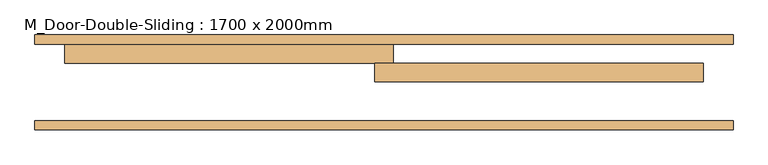
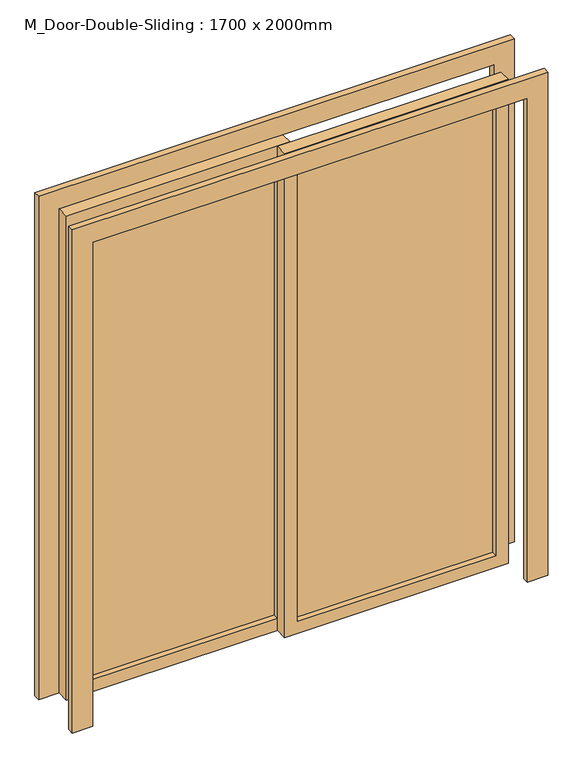
"""IFC4 building model written with IfcOpenShell, lengths in millimetres: door geometry, M_Door-Double-Sliding : 1700 x 2000mm."""

from ifc_helpers import new_model, si_unit, frame, origin, place, context, project, spatial, polyline, outline, extrude, source, transform, mapped, element, save


def m_door_double_sliding_1700_x_2000mm_96dae475(model_context):
    return source(origin(), model_context, "Body", "SweptSolid", [
        extrude(outline(polyline([(0.0, -930.0), (0.0, -850.0), (2000.0, -850.0), (2000.0, 850.0), (0.0, 850.0), (0.0, 930.0), (2080.0, 930.0), (2080.0, -930.0), (0.0, -930.0)])), frame((0.0, 0.4, 0.0), z_axis=(0.0, 1.0, 0.0), x_axis=(0.0, 0.0, 1.0)), (0.0, 0.0, 1.0), 25.0),
        extrude(outline(polyline([(0.0, 930.0), (2080.0, 930.0), (2080.0, -930.0), (0.0, -930.0), (0.0, -850.0), (2000.0, -850.0), (2000.0, 850.0), (0.0, 850.0), (0.0, 930.0)])), frame((0.0, 228.6, 0.0), z_axis=(0.0, 1.0, 0.0), x_axis=(0.0, 0.0, 1.0)), (0.0, 0.0, 1.0), 25.0),
        extrude(outline(polyline([(2000.0, -25.0), (0.0, -25.0), (0.0, 850.0), (2000.0, 850.0), (2000.0, -25.0)]), holes=[polyline([(1950.0, 25.0), (1950.0, 800.0), (50.0, 800.0), (50.0, 25.0), (1950.0, 25.0)])]), frame((0.0, 128.6, 0.0), z_axis=(0.0, 1.0, 0.0), x_axis=(0.0, 0.0, 1.0)), (0.0, 0.0, 1.0), 50.0),
        extrude(outline(polyline([(2000.0, 25.0), (2000.0, -850.0), (0.0, -850.0), (0.0, 25.0), (2000.0, 25.0)]), holes=[polyline([(1950.0, -25.0), (50.0, -25.0), (50.0, -800.0), (1950.0, -800.0), (1950.0, -25.0)])]), frame((0.0, 178.6, 0.0), z_axis=(0.0, 1.0, 0.0), x_axis=(0.0, 0.0, 1.0)), (0.0, 0.0, 1.0), 50.0),
        extrude(outline(polyline([(25.0, 156.775), (800.0, 156.775), (800.0, 150.425), (25.0, 150.425), (25.0, 156.775)])), frame((0.0, 0.0, 50.0), z_axis=(0.0, 0.0, 1.0), x_axis=(1.0, 0.0, 0.0)), (0.0, 0.0, 1.0), 1900.0),
        extrude(outline(polyline([(-25.0, 200.025), (-800.0, 200.025), (-800.0, 206.375), (-25.0, 206.375), (-25.0, 200.025)])), frame((0.0, 0.0, 50.0), z_axis=(0.0, 0.0, 1.0), x_axis=(1.0, 0.0, 0.0)), (0.0, 0.0, 1.0), 1900.0),
    ])


if __name__ == "__main__":
    model = new_model("IFC4")
    model_context = context("Model", 3, world=origin())
    ifc_project = project(units=[si_unit("LENGTHUNIT", "METRE", prefix="MILLI")], contexts=[model_context])
    site = spatial("IfcSite", under=ifc_project)
    building = spatial("IfcBuilding", under=site)
    placement = place(None, origin())
    m_door_double_sliding_1700_x_2000mm_shape = m_door_double_sliding_1700_x_2000mm_96dae475(model_context)
    element("IfcDoor", 1, ObjectType="M_Door-Double-Sliding : 1700 x 2000mm", at=placement, inside=building, context=model_context, shape_type="MappedRepresentation", body=[
        mapped(m_door_double_sliding_1700_x_2000mm_shape, transform((0.0, 0.0, 0.0), x_axis=(1.0, 0.0, 0.0), y_axis=(0.0, 1.0, 0.0), z_axis=(0.0, 0.0, 1.0))),
    ])
    save(model, "model.ifc")

# Revit data of these elements
# Type "M_Door-Double-Sliding : 1700 x 2000mm"
#   Type Mark = "11"
#   Construction Type Id = "opn-d45"
#   Assembly Code = "C1020"
#   Analytic Construction = "Wood frame, double glass door "
#   Thickness = 0' - 1.9685"
#   Thermal Resistance (R) = 0.31964 (m²·K)/W
#   Heat Transfer Coefficient (U) = 3.12872 W/(m²·K)
#   Height = 6' - 6.74016"
#   Rail Width = 0' - 1.9685"
#   Stiles = 0' - 1.9685"
#   Trim Projection Ext = 0' - 0.98425"
#   Trim Projection Int = 0' - 0.98425"
#   Trim Width = 0' - 3.14961"
#   Width = 5' - 6.92913"
#   Glazing = Glass
#   Panel Material = Wood - Birch - Solid Stained Light Low Gloss
#   Trim Material = Paint - Sienna
#   Visual Light Transmittance = 0
#   Solar Heat Gain Coefficient = 0
#   Function = (empty or 0)
#   Wall Closure = (empty or 0)
# Element 1 (IfcDoor, "M_Door-Double-Sliding : 1700 x 2000mm")
#   Materials on its faces: "Paint - Sienna", "Wood - Birch - Solid Stained Light Low Gloss", "Glass"
# Materials
#   "Glass": class "Glass", colour RGB 0 128 192, transparency 0.75, Description = "Soda Lime Glass", Cost = 0
#   "Wood - Birch - Solid Stained Light Low Gloss": class "Wood", colour RGB 210 159 95, transparency 0, Cost = 0
#   "Paint - Sienna": class "Miscellaneous", colour RGB 118 70 51, transparency 0, Cost = 0
